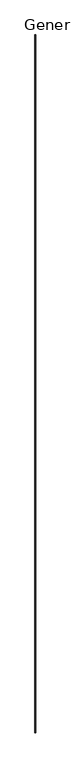
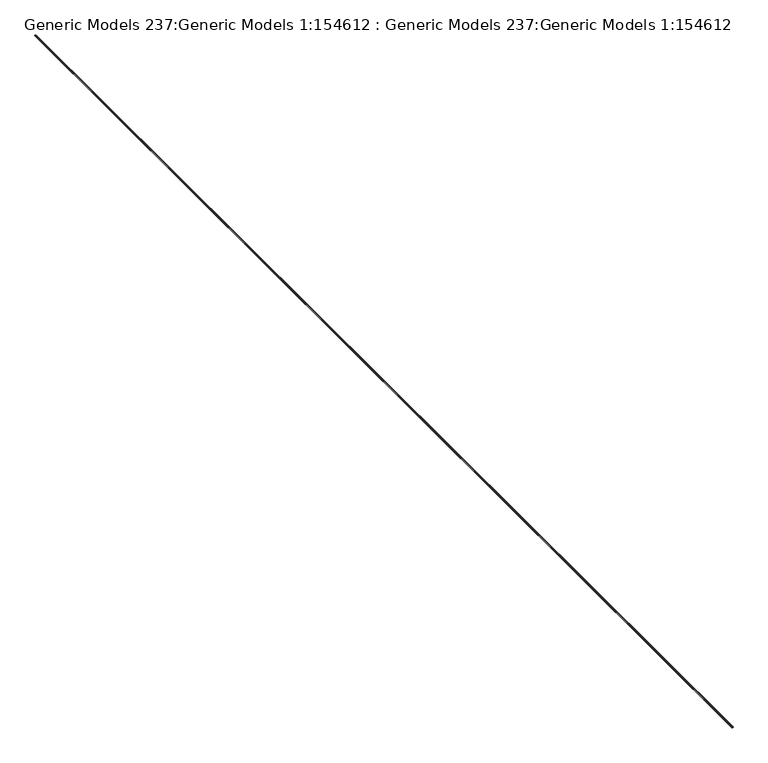
"""IFC4 building model written with IfcOpenShell, lengths in millimetres: proxy geometry, Generic Models 237:Generic Models 1:154612 : Generic Models 237:Generic Models 1:154612."""

from ifc_helpers import new_model, si_unit, point, frame, frame_2d, origin, place, context, project, spatial, polyline, circle_curve, trimmed, segment, composite_curve, outline, extrude, source, transform, mapped, element, save


def generic_models_237_generic_models_1_154612_generic_models_447ea2a8(model_context):
    return source(origin(), model_context, "Body", "SweptSolid", [
        extrude(outline(composite_curve([segment(trimmed(circle_curve(frame_2d((2942.3675253, 1476.3261519)), 6.4650413), [point((2947.1300253, 1480.6982627))], [point((2937.6050253, 1480.6982627))], True, "CARTESIAN"), True, "CONTINUOUS"), segment(polyline([(2937.6050253, 1480.6982627), (2937.6050253, 1485.4607627)]), True, "CONTINUOUS"), segment(trimmed(circle_curve(frame_2d((2942.3675253, 1481.0886519)), 6.4650413), [point((2937.6050253, 1485.4607627))], [point((2939.5110132, 1486.8884016))], False, "CARTESIAN"), True, "CONTINUOUS"), segment(polyline([(2939.5110132, 1486.8884016), (2938.7567788, 1487.9463145), (2938.1722903, 1489.2232154), (2937.7850254, 1490.6590755), (2937.6131898, 1492.1863931), (2937.6648617, 1493.7333671), (2937.937612, 1495.2272722), (2938.4186184, 1496.5978779), (2939.0852681, 1497.7807503), (2939.906221, 1498.7202809), (2940.842883, 1499.3723012), (2941.8512205, 1499.7061589), (2942.8838302, 1499.7061589), (2943.8921676, 1499.3723012), (2944.8288297, 1498.7202809), (2945.6497826, 1497.7807503), (2946.3164322, 1496.5978779), (2946.7974386, 1495.2272722), (2947.070189, 1493.7333671), (2947.1218609, 1492.1863931), (2946.9500253, 1490.6590755), (2946.5627603, 1489.2232154), (2945.9782719, 1487.9463145), (2945.2240375, 1486.8884016)]), True, "CONTINUOUS"), segment(trimmed(circle_curve(frame_2d((2942.3675253, 1481.0886519)), 6.4650413), [point((2945.2240375, 1486.8884016))], [point((2947.1300253, 1485.4607627))], False, "CARTESIAN"), True, "CONTINUOUS"), segment(polyline([(2947.1300253, 1485.4607627), (2947.1300253, 1480.6982627)]), True, "CONTINUOUS")], self_intersect=False)), frame((0.0, -7711.8185138, 0.0), z_axis=(0.0, 1.0, 0.0), x_axis=(0.0, 0.0, 1.0)), (0.0, 0.0, 1.0), 19050.0),
    ])


if __name__ == "__main__":
    model = new_model("IFC4")
    model_context = context("Model", 3, world=origin())
    ifc_project = project(units=[si_unit("LENGTHUNIT", "METRE", prefix="MILLI")], contexts=[model_context])
    site = spatial("IfcSite", under=ifc_project)
    building = spatial("IfcBuilding", under=site)
    placement = place(None, origin())
    generic_models_237_generic_models_1_154612_generic_models_shape = generic_models_237_generic_models_1_154612_generic_models_447ea2a8(model_context)
    element("IfcBuildingElementProxy", 1, Name="Generic Models 237:Generic Models 1:154612 : Generic Models 237:Generic Models 1:154612", ObjectType="Generic Models 237:Generic Models 1:154612 : Generic Models 237:Generic Models 1:154612", at=placement, inside=building, context=model_context, shape_type="MappedRepresentation", body=[
        mapped(generic_models_237_generic_models_1_154612_generic_models_shape, transform((0.0, 0.0, 0.0), x_axis=(1.0, 0.0, 0.0), y_axis=(0.0, 1.0, 0.0), z_axis=(0.0, 0.0, 1.0))),
    ])
    save(model, "model.ifc")

# Revit data of these elements
# Type "Generic Models 237:Generic Models 1:154612 : Generic Models 237:Generic Models 1:154612"
#   NameOverride = "Generic Models 237:Generic Models 1:154612"
#   ObjectTypeOverride = "Generic Models 237:Generic Models 1"
#   Reference = "Generic Models 1"
#   Category = "Generic Models"
#   Tag = "154612"
# Element 1 (IfcBuildingElementProxy, "Generic Models 237:Generic Models 1:154612 : Generic Models 237:Generic Models 1:154612")
#   Materials on its faces: "_SEALANT AND BACKROD, IF NECESSARY 12051"
# Materials
#   "_SEALANT AND BACKROD, IF NECESSARY 12051": class "Unassigned", colour RGB 190 220 196, transparency 0
